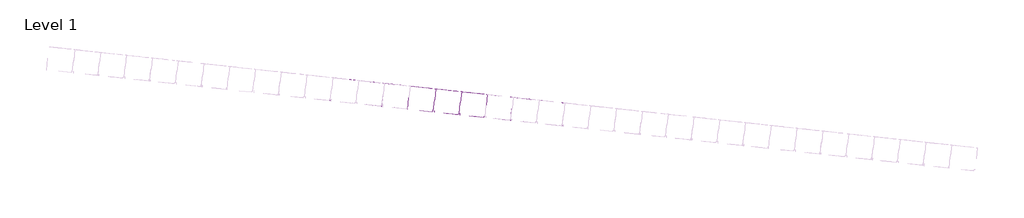
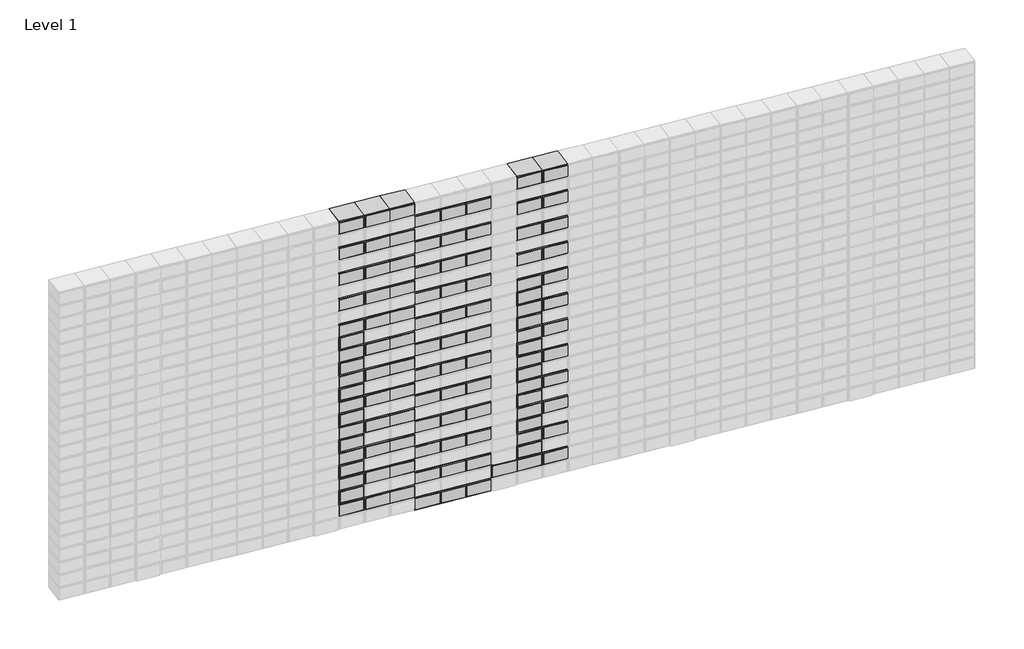
# One storey, part 14 of 18: 111 proxies.
"""IFC4 building model written with IfcOpenShell, lengths in millimetres."""

import ifcopenshell
import ifcopenshell.guid

model = None  # the IFC model being written
_history = None  # IfcOwnerHistory: only IFC2X3 demands one
_inside = {}  # id of a spatial element -> (the spatial element, [elements in it])
_under = {}  # id of a project, library or spatial element -> (it, [spatial elements below it])
_declared = {}  # id of a project -> (the project, [libraries it declares])
_typed = {}  # id of a type object -> (the type object, [elements of that type])
_made_of = {}  # id of a material, layer set ... -> (it, [elements and type objects made of it])


def new_model(schema):
    """Start an empty IFC model of exactly this schema.

    Asked for "IFC4X3", IfcOpenShell would pick the latest addendum, in which some entities
    have other attributes; the version numbers below select the first issue.
    IFC2X3 requires an IfcOwnerHistory on every rooted entity: one is made here for all.
    """
    global model, _history
    if schema == "IFC4X3":
        model = ifcopenshell.file(schema_version=(4, 3, 0, 0))
    else:
        model = ifcopenshell.file(schema=schema)
    _inside.clear()
    _under.clear()
    _declared.clear()
    _typed.clear()
    _made_of.clear()
    _history = None
    if model.schema == "IFC2X3":
        org = make("IfcOrganization", Name="unknown")
        user = make(
            "IfcPersonAndOrganization",
            ThePerson=make("IfcPerson", FamilyName="unknown"),
            TheOrganization=org,
        )
        app = make(
            "IfcApplication",
            ApplicationDeveloper=org,
            Version="unknown",
            ApplicationFullName="unknown",
            ApplicationIdentifier="unknown",
        )
        _history = make(
            "IfcOwnerHistory",
            OwningUser=user,
            OwningApplication=app,
            ChangeAction="ADDED",
            CreationDate=0,
        )
    return model


def make(cls, **values):
    """One entity of the class cls with the attributes given. An attribute that is None is left unset."""
    return model.create_entity(
        cls, **{name: value for name, value in values.items() if value is not None}
    )


def rooted(cls, **values):
    """An entity with a GlobalId (a new one), such as an element, a storey or a relation."""
    return make(cls, GlobalId=ifcopenshell.guid.new(), OwnerHistory=_history, **values)


def si_unit(unit_type, name, prefix=None):
    """IfcSIUnit, for example si_unit("LENGTHUNIT", "METRE", prefix="MILLI")."""
    return make("IfcSIUnit", UnitType=unit_type, Prefix=prefix, Name=name)


def assignment(units):
    """IfcUnitAssignment: the units of a project."""
    return None if units is None else make("IfcUnitAssignment", Units=units)


def point(xyz):
    """IfcCartesianPoint."""
    return None if xyz is None else make("IfcCartesianPoint", Coordinates=xyz)


def direction(xyz):
    """IfcDirection."""
    return None if xyz is None else make("IfcDirection", DirectionRatios=xyz)


def frame(location, z_axis=None, x_axis=None):
    """IfcAxis2Placement3D, a coordinate frame: its origin and axes. An axis left out is left unset."""
    return make(
        "IfcAxis2Placement3D",
        Location=point(location),
        Axis=direction(z_axis),
        RefDirection=direction(x_axis),
    )


def origin():
    """The frame at (0, 0, 0) with its axes left unset."""
    return frame((0.0, 0.0, 0.0))


def origin_with_axes():
    """The frame at (0, 0, 0) with the z axis (0, 0, 1) and the x axis (1, 0, 0) written out."""
    return frame((0.0, 0.0, 0.0), z_axis=(0.0, 0.0, 1.0), x_axis=(1.0, 0.0, 0.0))


def place(relative_to, where):
    """IfcLocalPlacement: puts the frame where relative to a parent placement (None: the world)."""
    return make(
        "IfcLocalPlacement", PlacementRelTo=relative_to, RelativePlacement=where
    )


def context(
    kind, dimensions, precision=None, world=None, true_north=None, identifier=None
):
    """IfcGeometricRepresentationContext, for example the 3D "Model" context."""
    return make(
        "IfcGeometricRepresentationContext",
        ContextIdentifier=identifier,
        ContextType=kind,
        CoordinateSpaceDimension=dimensions,
        Precision=precision,
        WorldCoordinateSystem=world,
        TrueNorth=true_north,
    )


def project(units=None, contexts=None):
    """IfcProject with its units and contexts."""
    return rooted(
        "IfcProject",
        Name="project",
        RepresentationContexts=contexts,
        UnitsInContext=assignment(units),
    )


def spatial(cls, under=None, at=None, **own):
    """A site, building, storey or space (cls), placed at a placement, below another one or the project."""
    s = rooted(cls, ObjectPlacement=at, **own)
    if under is not None:
        _under.setdefault(under.id(), (under, []))[1].append(s)
    return s


def polyline(points):
    """IfcPolyline through the points."""
    return make("IfcPolyline", Points=[point(p) for p in points])


def outline(outer, holes=None, kind="AREA"):
    """IfcArbitraryClosedProfileDef: a profile drawn as a closed curve; with holes, ...WithVoids."""
    if holes is None:
        return make("IfcArbitraryClosedProfileDef", ProfileType=kind, OuterCurve=outer)
    return make(
        "IfcArbitraryProfileDefWithVoids",
        ProfileType=kind,
        OuterCurve=outer,
        InnerCurves=holes,
    )


def extrude(swept, where, along, depth):
    """IfcExtrudedAreaSolid: the profile swept, set in the frame where, extruded along a direction by depth."""
    return make(
        "IfcExtrudedAreaSolid",
        SweptArea=swept,
        Position=where,
        ExtrudedDirection=direction(along),
        Depth=depth,
    )


def shape(context_of_items, identifier, shape_type, items):
    """IfcShapeRepresentation: the items that make up one representation, for example the "Body"."""
    return make(
        "IfcShapeRepresentation",
        ContextOfItems=context_of_items,
        RepresentationIdentifier=identifier,
        RepresentationType=shape_type,
        Items=items,
    )


def source(mapping_origin, context_of_items, identifier, shape_type, items):
    """IfcRepresentationMap: a shape defined once, which mapped items show again and again."""
    return make(
        "IfcRepresentationMap",
        MappingOrigin=mapping_origin,
        MappedRepresentation=shape(context_of_items, identifier, shape_type, items),
    )


def transform(
    local_origin,
    x_axis=None,
    y_axis=None,
    z_axis=None,
    scale=None,
    scale2=None,
    scale3=None,
    uniform=True,
):
    """IfcCartesianTransformationOperator3D, or its non-uniform kind. x_axis, y_axis, z_axis: its Axis1, 2, 3."""
    if uniform:
        return make(
            "IfcCartesianTransformationOperator3D",
            Axis1=direction(x_axis),
            Axis2=direction(y_axis),
            LocalOrigin=point(local_origin),
            Scale=scale,
            Axis3=direction(z_axis),
        )
    return make(
        "IfcCartesianTransformationOperator3DnonUniform",
        Axis1=direction(x_axis),
        Axis2=direction(y_axis),
        LocalOrigin=point(local_origin),
        Scale=scale,
        Axis3=direction(z_axis),
        Scale2=scale2,
        Scale3=scale3,
    )


def mapped(mapping_source, mapping_target):
    """IfcMappedItem: shows the shape of a source again, moved by a transform."""
    return make(
        "IfcMappedItem", MappingSource=mapping_source, MappingTarget=mapping_target
    )


def made_of(thing, what):
    """Note that an element or type object is made of a material, layer set ...; save() writes the relation."""
    if what is not None:
        _made_of.setdefault(what.id(), (what, []))[1].append(thing)
    return thing


def element(
    cls,
    number,
    at=None,
    inside=None,
    cuts=None,
    type_object=None,
    material=None,
    context=None,
    identifier="Body",
    shape_type=None,
    held_by="IfcProductDefinitionShape",
    body=None,
    shapes=None,
    **own,
):
    """One element of the class cls, such as IfcWall. Its Tag is "e" and its number.

    at: its placement. inside: the storey or other place that contains it. cuts: it is an
    opening in that element (IfcRelVoidsElement). A single representation is given by context,
    identifier, shape_type and body (its items); several are given by shapes. held_by: the class
    of the entity that holds the representations. save() writes the other relations.
    """
    e = rooted(cls, Tag="e%d" % number, ObjectPlacement=at, **own)
    if body is not None:
        shapes = [shape(context, identifier, shape_type, body)]
    if shapes is not None:
        e.Representation = make(held_by, Representations=shapes)
    if inside is not None:
        _inside.setdefault(inside.id(), (inside, []))[1].append(e)
    if cuts is not None:
        rooted(
            "IfcRelVoidsElement", RelatingBuildingElement=cuts, RelatedOpeningElement=e
        )
    if type_object is not None:
        _typed.setdefault(type_object.id(), (type_object, []))[1].append(e)
    return made_of(e, material)


def aggregate(whole, parts):
    """IfcRelAggregates: a whole, such as a stair, and the parts it consists of."""
    return rooted("IfcRelAggregates", RelatingObject=whole, RelatedObjects=parts)


def save(model, path):
    """Write the relations noted so far, then the file.

    IfcRelAggregates (storeys below a building ...), IfcRelContainedInSpatialStructure (elements
    in a storey), IfcRelDefinesByType, IfcRelAssociatesMaterial and IfcRelDeclares: one each for
    every whole, place, type object, material and project.
    """
    for whole, parts in _under.values():
        aggregate(whole, parts)
    for where, things in _inside.values():
        rooted(
            "IfcRelContainedInSpatialStructure",
            RelatedElements=things,
            RelatingStructure=where,
        )
    for kind, things in _typed.values():
        rooted("IfcRelDefinesByType", RelatedObjects=things, RelatingType=kind)
    for what, things in _made_of.values():
        rooted("IfcRelAssociatesMaterial", RelatedObjects=things, RelatingMaterial=what)
    for by, libraries in _declared.values():
        rooted("IfcRelDeclares", RelatingContext=by, RelatedDefinitions=libraries)
    model.write(path)


def geel_a5fc7152(model_context):
    return source(origin(), model_context, "Body", "SweptSolid", [
        extrude(outline(polyline([(131.1871262, 51.8695461), (24.8461542, 24.0369432), (23.5801491, 28.8740117), (125.0840527, 55.4406095), (111.9430518, 105.6488784), (10.4391482, 79.0822806), (9.1731432, 83.919349), (115.5141152, 111.7519519), (131.1871262, 51.8695461)])), origin_with_axes(), (0.0, 0.0, 1.0), 95.0),
        extrude(outline(polyline([(111.9430518, 105.6488784), (125.0840527, 55.4406095), (23.5801491, 28.8740117), (10.4391482, 79.0822806), (111.9430518, 105.6488784)])), origin_with_axes(), (0.0, 0.0, 1.0), 100.0),
    ])


def geel_ff5a4212(model_context):
    return source(origin(), model_context, "Body", "SweptSolid", [
        extrude(outline(polyline([(24.8461542, 24.0369432), (9.1731432, 83.919349), (115.5141152, 111.7519519), (116.7801202, 106.9148835), (15.2762167, 80.3482856), (28.4172176, 30.1400167), (129.9211211, 56.7066146), (131.1871262, 51.8695461), (24.8461542, 24.0369432)])), origin_with_axes(), (0.0, 0.0, 1.0), 95.0),
        extrude(outline(polyline([(116.7801202, 106.9148835), (129.9211211, 56.7066146), (28.4172176, 30.1400167), (15.2762167, 80.3482856), (116.7801202, 106.9148835)])), origin_with_axes(), (0.0, 0.0, 1.0), 100.0),
    ])


def rood_14a66368(model_context):
    return source(origin(), model_context, "Body", "SweptSolid", [
        extrude(outline(polyline([(24.8461542, 24.0369432), (9.1731432, 83.919349), (115.5141152, 111.7519519), (131.1871262, 51.8695461), (24.8461542, 24.0369432)]), holes=[polyline([(125.0840527, 55.4406095), (111.9430518, 105.6488784), (15.2762167, 80.3482856), (28.4172176, 30.1400167), (125.0840527, 55.4406095)])]), origin_with_axes(), (0.0, 0.0, 1.0), 95.0),
        extrude(outline(polyline([(111.9430518, 105.6488784), (125.0840527, 55.4406095), (28.4172176, 30.1400167), (15.2762167, 80.3482856), (111.9430518, 105.6488784)])), origin_with_axes(), (0.0, 0.0, 1.0), 100.0),
    ])


model = new_model("IFC4")

# Units and contexts
model_context = context("Model", 3, world=origin())
ifc_project = project(units=[si_unit("LENGTHUNIT", "METRE", prefix="MILLI")], contexts=[model_context])

# Site, building, storey
site = spatial("IfcSite", under=ifc_project)
building = spatial("IfcBuilding", under=site)
storey = spatial("IfcBuildingStorey", under=building, Name="Level 1", Elevation=0.0)

# Proxies
placement = place(None, origin())
geel_shape = geel_a5fc7152(model_context)
element("IfcBuildingElementProxy", 1, Name="Geel", ObjectType="Geel", at=placement, inside=storey, context=model_context, shape_type="MappedRepresentation", body=[
    mapped(geel_shape, transform((10079.135101, -4407.170809, 2168.7358475), x_axis=(0.9617275503729381, -0.10473475661476775, -0.25320100633787634), y_axis=(0.2517127736886919, -0.02741220845642843, 0.9674136914420257), z_axis=(-0.1082626362860859, -0.9941223272738555, 0.0))),
])
element("IfcBuildingElementProxy", 2, Name="Geel", ObjectType="Geel", at=placement, inside=storey, context=model_context, shape_type="MappedRepresentation", body=[
    mapped(geel_shape, transform((10844.0731503, -4490.4746516, 2168.7358475), x_axis=(0.9617275503729374, -0.1047347566147725, -0.25320100633787673), y_axis=(0.25171277368869216, -0.02741220845642974, 0.9674136914420255), z_axis=(-0.10826263628609081, -0.9941223272738551, 0.0))),
])
element("IfcBuildingElementProxy", 3, Name="Geel", ObjectType="Geel", at=placement, inside=storey, context=model_context, shape_type="MappedRepresentation", body=[
    mapped(geel_shape, transform((10079.135101, -4407.170809, 2292.5348104), x_axis=(0.9617275503729381, -0.10473475661476775, -0.25320100633787634), y_axis=(0.2517127736886919, -0.02741220845642843, 0.9674136914420257), z_axis=(-0.1082626362860859, -0.9941223272738555, 0.0))),
])
element("IfcBuildingElementProxy", 4, Name="Geel", ObjectType="Geel", at=placement, inside=storey, context=model_context, shape_type="MappedRepresentation", body=[
    mapped(geel_shape, transform((10844.0731503, -4490.4746516, 2292.5348104), x_axis=(0.9617275503729374, -0.1047347566147725, -0.25320100633787673), y_axis=(0.25171277368869216, -0.02741220845642974, 0.9674136914420255), z_axis=(-0.10826263628609081, -0.9941223272738551, 0.0))),
])
element("IfcBuildingElementProxy", 5, Name="Geel", ObjectType="Geel", at=placement, inside=storey, context=model_context, shape_type="MappedRepresentation", body=[
    mapped(geel_shape, transform((10079.135101, -4407.170809, 2416.3337732), x_axis=(0.961727550372939, -0.10473475661476785, -0.2532010063378727), y_axis=(0.2517127736886882, -0.02741220845642804, 0.9674136914420266), z_axis=(-0.1082626362860859, -0.9941223272738555, 0.0))),
])
element("IfcBuildingElementProxy", 6, Name="Geel", ObjectType="Geel", at=placement, inside=storey, context=model_context, shape_type="MappedRepresentation", body=[
    mapped(geel_shape, transform((10844.0731503, -4490.4746516, 2416.3337732), x_axis=(0.9617275503729384, -0.1047347566147726, -0.25320100633787307), y_axis=(0.25171277368868855, -0.02741220845642934, 0.9674136914420265), z_axis=(-0.10826263628609081, -0.994122327273855, 0.0))),
])
element("IfcBuildingElementProxy", 7, Name="Geel", ObjectType="Geel", at=placement, inside=storey, context=model_context, shape_type="MappedRepresentation", body=[
    mapped(geel_shape, transform((10079.135101, -4407.170809, 2540.132736), x_axis=(0.9617275503729381, -0.10473475661476775, -0.25320100633787634), y_axis=(0.2517127736886919, -0.02741220845642843, 0.9674136914420257), z_axis=(-0.1082626362860859, -0.9941223272738555, 0.0))),
])
element("IfcBuildingElementProxy", 8, Name="Geel", ObjectType="Geel", at=placement, inside=storey, context=model_context, shape_type="MappedRepresentation", body=[
    mapped(geel_shape, transform((10844.0731503, -4490.4746516, 2540.132736), x_axis=(0.9617275503729374, -0.1047347566147725, -0.25320100633787673), y_axis=(0.25171277368869216, -0.02741220845642974, 0.9674136914420255), z_axis=(-0.10826263628609081, -0.9941223272738551, 0.0))),
])
element("IfcBuildingElementProxy", 9, Name="Geel", ObjectType="Geel", at=placement, inside=storey, context=model_context, shape_type="MappedRepresentation", body=[
    mapped(geel_shape, transform((10079.135101, -4407.170809, 2663.9316989), x_axis=(0.9617275503729381, -0.10473475661476775, -0.25320100633787634), y_axis=(0.2517127736886919, -0.02741220845642843, 0.9674136914420257), z_axis=(-0.1082626362860859, -0.9941223272738555, 0.0))),
])
element("IfcBuildingElementProxy", 10, Name="Geel", ObjectType="Geel", at=placement, inside=storey, context=model_context, shape_type="MappedRepresentation", body=[
    mapped(geel_shape, transform((10844.0731503, -4490.4746516, 2663.9316989), x_axis=(0.9617275503729374, -0.1047347566147725, -0.25320100633787673), y_axis=(0.25171277368869216, -0.02741220845642974, 0.9674136914420255), z_axis=(-0.10826263628609081, -0.9941223272738551, 0.0))),
])
element("IfcBuildingElementProxy", 11, Name="Geel", ObjectType="Geel", at=placement, inside=storey, context=model_context, shape_type="MappedRepresentation", body=[
    mapped(geel_shape, transform((10079.135101, -4407.170809, 2787.7306617), x_axis=(0.9617275503729381, -0.10473475661476775, -0.25320100633787634), y_axis=(0.2517127736886919, -0.02741220845642843, 0.9674136914420257), z_axis=(-0.1082626362860859, -0.9941223272738555, 0.0))),
])
element("IfcBuildingElementProxy", 12, Name="Geel", ObjectType="Geel", at=placement, inside=storey, context=model_context, shape_type="MappedRepresentation", body=[
    mapped(geel_shape, transform((10844.0731503, -4490.4746516, 2787.7306617), x_axis=(0.9617275503729374, -0.1047347566147725, -0.25320100633787673), y_axis=(0.25171277368869216, -0.02741220845642974, 0.9674136914420255), z_axis=(-0.10826263628609081, -0.9941223272738551, 0.0))),
])
element("IfcBuildingElementProxy", 13, Name="Geel", ObjectType="Geel", at=placement, inside=storey, context=model_context, shape_type="MappedRepresentation", body=[
    mapped(geel_shape, transform((10079.135101, -4407.170809, 2911.5296245), x_axis=(0.9617275503729381, -0.10473475661476775, -0.25320100633787634), y_axis=(0.2517127736886919, -0.02741220845642843, 0.9674136914420257), z_axis=(-0.1082626362860859, -0.9941223272738555, 0.0))),
])
element("IfcBuildingElementProxy", 14, Name="Geel", ObjectType="Geel", at=placement, inside=storey, context=model_context, shape_type="MappedRepresentation", body=[
    mapped(geel_shape, transform((10844.0731503, -4490.4746516, 2911.5296245), x_axis=(0.9617275503729374, -0.1047347566147725, -0.25320100633787673), y_axis=(0.25171277368869216, -0.02741220845642974, 0.9674136914420255), z_axis=(-0.10826263628609081, -0.9941223272738551, 0.0))),
])
element("IfcBuildingElementProxy", 15, Name="Geel", ObjectType="Geel", at=placement, inside=storey, context=model_context, shape_type="MappedRepresentation", body=[
    mapped(geel_shape, transform((10079.135101, -4407.170809, 3035.3285874), x_axis=(0.9617275503729381, -0.10473475661476775, -0.25320100633787634), y_axis=(0.2517127736886919, -0.02741220845642843, 0.9674136914420257), z_axis=(-0.1082626362860859, -0.9941223272738555, 0.0))),
])
element("IfcBuildingElementProxy", 16, Name="Geel", ObjectType="Geel", at=placement, inside=storey, context=model_context, shape_type="MappedRepresentation", body=[
    mapped(geel_shape, transform((10844.0731503, -4490.4746516, 3035.3285874), x_axis=(0.9617275503729374, -0.1047347566147725, -0.25320100633787673), y_axis=(0.25171277368869216, -0.02741220845642974, 0.9674136914420255), z_axis=(-0.10826263628609081, -0.9941223272738551, 0.0))),
])
element("IfcBuildingElementProxy", 17, Name="Geel", ObjectType="Geel", at=placement, inside=storey, context=model_context, shape_type="MappedRepresentation", body=[
    mapped(geel_shape, transform((10079.135101, -4407.170809, 3159.1275502), x_axis=(0.9617275503729381, -0.10473475661476775, -0.25320100633787634), y_axis=(0.2517127736886919, -0.02741220845642843, 0.9674136914420257), z_axis=(-0.1082626362860859, -0.9941223272738555, 0.0))),
])
element("IfcBuildingElementProxy", 18, Name="Geel", ObjectType="Geel", at=placement, inside=storey, context=model_context, shape_type="MappedRepresentation", body=[
    mapped(geel_shape, transform((10844.0731503, -4490.4746516, 3159.1275502), x_axis=(0.9617275503729374, -0.1047347566147725, -0.25320100633787673), y_axis=(0.25171277368869216, -0.02741220845642974, 0.9674136914420255), z_axis=(-0.10826263628609081, -0.9941223272738551, 0.0))),
])
element("IfcBuildingElementProxy", 19, Name="Geel", ObjectType="Geel", at=placement, inside=storey, context=model_context, shape_type="MappedRepresentation", body=[
    mapped(geel_shape, transform((10079.135101, -4407.170809, 3282.926513), x_axis=(0.9617275503729381, -0.10473475661476775, -0.25320100633787634), y_axis=(0.2517127736886919, -0.02741220845642843, 0.9674136914420257), z_axis=(-0.1082626362860859, -0.9941223272738555, 0.0))),
])
element("IfcBuildingElementProxy", 20, Name="Geel", ObjectType="Geel", at=placement, inside=storey, context=model_context, shape_type="MappedRepresentation", body=[
    mapped(geel_shape, transform((10844.0731503, -4490.4746516, 3282.926513), x_axis=(0.9617275503729374, -0.1047347566147725, -0.25320100633787673), y_axis=(0.25171277368869216, -0.02741220845642974, 0.9674136914420255), z_axis=(-0.10826263628609081, -0.9941223272738551, 0.0))),
])
element("IfcBuildingElementProxy", 21, Name="Geel", ObjectType="Geel", at=placement, inside=storey, context=model_context, shape_type="MappedRepresentation", body=[
    mapped(geel_shape, transform((10079.135101, -4407.170809, 3406.7254759), x_axis=(0.9617275503729381, -0.10473475661476775, -0.25320100633787634), y_axis=(0.2517127736886919, -0.02741220845642843, 0.9674136914420257), z_axis=(-0.1082626362860859, -0.9941223272738555, 0.0))),
])
element("IfcBuildingElementProxy", 22, Name="Geel", ObjectType="Geel", at=placement, inside=storey, context=model_context, shape_type="MappedRepresentation", body=[
    mapped(geel_shape, transform((10844.0731503, -4490.4746516, 3406.7254759), x_axis=(0.9617275503729374, -0.1047347566147725, -0.25320100633787673), y_axis=(0.25171277368869216, -0.02741220845642974, 0.9674136914420255), z_axis=(-0.10826263628609081, -0.9941223272738551, 0.0))),
])
element("IfcBuildingElementProxy", 23, Name="Geel", ObjectType="Geel", at=placement, inside=storey, context=model_context, shape_type="MappedRepresentation", body=[
    mapped(geel_shape, transform((10079.135101, -4407.170809, 2044.9368847), x_axis=(0.961727550372939, -0.10473475661476785, -0.2532010063378727), y_axis=(0.2517127736886882, -0.02741220845642804, 0.9674136914420266), z_axis=(-0.1082626362860859, -0.9941223272738555, 0.0))),
])
element("IfcBuildingElementProxy", 24, Name="Geel", ObjectType="Geel", at=placement, inside=storey, context=model_context, shape_type="MappedRepresentation", body=[
    mapped(geel_shape, transform((10844.0731503, -4490.4746516, 2044.9368847), x_axis=(0.9617275503729384, -0.1047347566147726, -0.25320100633787307), y_axis=(0.25171277368868855, -0.02741220845642934, 0.9674136914420265), z_axis=(-0.10826263628609081, -0.994122327273855, 0.0))),
])
element("IfcBuildingElementProxy", 25, Name="Geel", ObjectType="Geel", at=placement, inside=storey, context=model_context, shape_type="MappedRepresentation", body=[
    mapped(geel_shape, transform((10297.6888294, -4430.9719069, 2168.7358475), x_axis=(0.9617275503729374, -0.1047347566147725, -0.25320100633787673), y_axis=(0.25171277368869216, -0.02741220845642974, 0.9674136914420255), z_axis=(-0.10826263628609081, -0.9941223272738551, 0.0))),
])
element("IfcBuildingElementProxy", 26, Name="Geel", ObjectType="Geel", at=placement, inside=storey, context=model_context, shape_type="MappedRepresentation", body=[
    mapped(geel_shape, transform((10297.6888294, -4430.9719069, 2292.5348104), x_axis=(0.9617275503729374, -0.1047347566147725, -0.25320100633787673), y_axis=(0.25171277368869216, -0.02741220845642974, 0.9674136914420255), z_axis=(-0.10826263628609081, -0.9941223272738551, 0.0))),
])
element("IfcBuildingElementProxy", 27, Name="Geel", ObjectType="Geel", at=placement, inside=storey, context=model_context, shape_type="MappedRepresentation", body=[
    mapped(geel_shape, transform((10297.6888294, -4430.9719069, 2416.3337732), x_axis=(0.9617275503729384, -0.1047347566147726, -0.25320100633787307), y_axis=(0.25171277368868855, -0.02741220845642934, 0.9674136914420265), z_axis=(-0.10826263628609081, -0.994122327273855, 0.0))),
])
element("IfcBuildingElementProxy", 28, Name="Geel", ObjectType="Geel", at=placement, inside=storey, context=model_context, shape_type="MappedRepresentation", body=[
    mapped(geel_shape, transform((10297.6888294, -4430.9719069, 2540.132736), x_axis=(0.9617275503729374, -0.1047347566147725, -0.25320100633787673), y_axis=(0.25171277368869216, -0.02741220845642974, 0.9674136914420255), z_axis=(-0.10826263628609081, -0.9941223272738551, 0.0))),
])
element("IfcBuildingElementProxy", 29, Name="Geel", ObjectType="Geel", at=placement, inside=storey, context=model_context, shape_type="MappedRepresentation", body=[
    mapped(geel_shape, transform((10297.6888294, -4430.9719069, 2663.9316989), x_axis=(0.9617275503729374, -0.1047347566147725, -0.25320100633787673), y_axis=(0.25171277368869216, -0.02741220845642974, 0.9674136914420255), z_axis=(-0.10826263628609081, -0.9941223272738551, 0.0))),
])
element("IfcBuildingElementProxy", 30, Name="Geel", ObjectType="Geel", at=placement, inside=storey, context=model_context, shape_type="MappedRepresentation", body=[
    mapped(geel_shape, transform((10297.6888294, -4430.9719069, 2787.7306617), x_axis=(0.9617275503729374, -0.1047347566147725, -0.25320100633787673), y_axis=(0.25171277368869216, -0.02741220845642974, 0.9674136914420255), z_axis=(-0.10826263628609081, -0.9941223272738551, 0.0))),
])
element("IfcBuildingElementProxy", 31, Name="Geel", ObjectType="Geel", at=placement, inside=storey, context=model_context, shape_type="MappedRepresentation", body=[
    mapped(geel_shape, transform((10297.6888294, -4430.9719069, 2911.5296245), x_axis=(0.9617275503729374, -0.1047347566147725, -0.25320100633787673), y_axis=(0.25171277368869216, -0.02741220845642974, 0.9674136914420255), z_axis=(-0.10826263628609081, -0.9941223272738551, 0.0))),
])
element("IfcBuildingElementProxy", 32, Name="Geel", ObjectType="Geel", at=placement, inside=storey, context=model_context, shape_type="MappedRepresentation", body=[
    mapped(geel_shape, transform((10297.6888294, -4430.9719069, 3035.3285874), x_axis=(0.9617275503729374, -0.1047347566147725, -0.25320100633787673), y_axis=(0.25171277368869216, -0.02741220845642974, 0.9674136914420255), z_axis=(-0.10826263628609081, -0.9941223272738551, 0.0))),
])
element("IfcBuildingElementProxy", 33, Name="Geel", ObjectType="Geel", at=placement, inside=storey, context=model_context, shape_type="MappedRepresentation", body=[
    mapped(geel_shape, transform((10297.6888294, -4430.9719069, 3159.1275502), x_axis=(0.9617275503729374, -0.1047347566147725, -0.25320100633787673), y_axis=(0.25171277368869216, -0.02741220845642974, 0.9674136914420255), z_axis=(-0.10826263628609081, -0.9941223272738551, 0.0))),
])
element("IfcBuildingElementProxy", 34, Name="Geel", ObjectType="Geel", at=placement, inside=storey, context=model_context, shape_type="MappedRepresentation", body=[
    mapped(geel_shape, transform((10297.6888294, -4430.9719069, 3282.926513), x_axis=(0.9617275503729374, -0.1047347566147725, -0.25320100633787673), y_axis=(0.25171277368869216, -0.02741220845642974, 0.9674136914420255), z_axis=(-0.10826263628609081, -0.9941223272738551, 0.0))),
])
element("IfcBuildingElementProxy", 35, Name="Geel", ObjectType="Geel", at=placement, inside=storey, context=model_context, shape_type="MappedRepresentation", body=[
    mapped(geel_shape, transform((10297.6888294, -4430.9719069, 3406.7254759), x_axis=(0.9617275503729374, -0.1047347566147725, -0.25320100633787673), y_axis=(0.25171277368869216, -0.02741220845642974, 0.9674136914420255), z_axis=(-0.10826263628609081, -0.9941223272738551, 0.0))),
])
element("IfcBuildingElementProxy", 36, Name="Geel", ObjectType="Geel", at=placement, inside=storey, context=model_context, shape_type="MappedRepresentation", body=[
    mapped(geel_shape, transform((10297.6888294, -4430.9719069, 2044.9368847), x_axis=(0.9617275503729384, -0.1047347566147726, -0.25320100633787307), y_axis=(0.25171277368868855, -0.02741220845642934, 0.9674136914420265), z_axis=(-0.10826263628609081, -0.994122327273855, 0.0))),
])
geel_2_shape = geel_ff5a4212(model_context)
element("IfcBuildingElementProxy", 37, Name="Geel", ObjectType="Geel", at=placement, inside=storey, context=model_context, shape_type="MappedRepresentation", body=[
    mapped(geel_2_shape, transform((10734.7962861, -4478.5741026, 2044.9368847), x_axis=(0.961727550372943, -0.10473475661477039, -0.25320100633785686), y_axis=(0.25171277368867245, -0.02741220845642689, 0.9674136914420308), z_axis=(-0.10826263628608805, -0.9941223272738553, 0.0))),
])
element("IfcBuildingElementProxy", 38, Name="Geel", ObjectType="Geel", at=placement, inside=storey, context=model_context, shape_type="MappedRepresentation", body=[
    mapped(geel_2_shape, transform((10188.4119652, -4419.071358, 2168.7358475), x_axis=(0.9617275503729416, -0.10473475661477503, -0.2532010063378606), y_axis=(0.25171277368867595, -0.027412208456428513, 0.9674136914420297), z_axis=(-0.10826263628609296, -0.9941223272738547, 0.0))),
])
element("IfcBuildingElementProxy", 39, Name="Geel", ObjectType="Geel", at=placement, inside=storey, context=model_context, shape_type="MappedRepresentation", body=[
    mapped(geel_2_shape, transform((10953.3500145, -4502.3752005, 2168.7358475), x_axis=(0.961727550372942, -0.10473475661477023, -0.25320100633786047), y_axis=(0.2517127736886762, -0.02741220845642727, 0.9674136914420297), z_axis=(-0.10826263628608801, -0.9941223272738554, 0.0))),
])
element("IfcBuildingElementProxy", 40, Name="Geel", ObjectType="Geel", at=placement, inside=storey, context=model_context, shape_type="MappedRepresentation", body=[
    mapped(geel_2_shape, transform((10188.4119652, -4419.071358, 2292.5348104), x_axis=(0.9617275503729416, -0.10473475661477503, -0.2532010063378606), y_axis=(0.25171277368867595, -0.027412208456428513, 0.9674136914420297), z_axis=(-0.10826263628609296, -0.9941223272738547, 0.0))),
])
element("IfcBuildingElementProxy", 41, Name="Geel", ObjectType="Geel", at=placement, inside=storey, context=model_context, shape_type="MappedRepresentation", body=[
    mapped(geel_2_shape, transform((10953.3500145, -4502.3752005, 2292.5348104), x_axis=(0.961727550372942, -0.10473475661477023, -0.25320100633786047), y_axis=(0.2517127736886762, -0.02741220845642727, 0.9674136914420297), z_axis=(-0.10826263628608801, -0.9941223272738554, 0.0))),
])
element("IfcBuildingElementProxy", 42, Name="Geel", ObjectType="Geel", at=placement, inside=storey, context=model_context, shape_type="MappedRepresentation", body=[
    mapped(geel_2_shape, transform((10188.4119652, -4419.071358, 2416.3337732), x_axis=(0.9617275503729426, -0.10473475661477512, -0.253201006337857), y_axis=(0.2517127736886723, -0.027412208456428104, 0.9674136914420308), z_axis=(-0.10826263628609295, -0.9941223272738549, 0.0))),
])
element("IfcBuildingElementProxy", 43, Name="Geel", ObjectType="Geel", at=placement, inside=storey, context=model_context, shape_type="MappedRepresentation", body=[
    mapped(geel_2_shape, transform((10953.3500145, -4502.3752005, 2416.3337732), x_axis=(0.961727550372943, -0.10473475661477034, -0.25320100633785686), y_axis=(0.25171277368867245, -0.027412208456426876, 0.9674136914420308), z_axis=(-0.10826263628608801, -0.9941223272738553, 0.0))),
])
element("IfcBuildingElementProxy", 44, Name="Geel", ObjectType="Geel", at=placement, inside=storey, context=model_context, shape_type="MappedRepresentation", body=[
    mapped(geel_2_shape, transform((10188.4119652, -4419.071358, 2540.132736), x_axis=(0.9617275503729416, -0.10473475661477503, -0.2532010063378606), y_axis=(0.25171277368867595, -0.027412208456428513, 0.9674136914420297), z_axis=(-0.10826263628609296, -0.9941223272738547, 0.0))),
])
element("IfcBuildingElementProxy", 45, Name="Geel", ObjectType="Geel", at=placement, inside=storey, context=model_context, shape_type="MappedRepresentation", body=[
    mapped(geel_2_shape, transform((10953.3500145, -4502.3752005, 2540.132736), x_axis=(0.961727550372942, -0.10473475661477023, -0.25320100633786047), y_axis=(0.2517127736886762, -0.02741220845642727, 0.9674136914420297), z_axis=(-0.10826263628608801, -0.9941223272738554, 0.0))),
])
element("IfcBuildingElementProxy", 46, Name="Geel", ObjectType="Geel", at=placement, inside=storey, context=model_context, shape_type="MappedRepresentation", body=[
    mapped(geel_2_shape, transform((10188.4119652, -4419.071358, 2663.9316989), x_axis=(0.9617275503729416, -0.10473475661477503, -0.2532010063378606), y_axis=(0.25171277368867595, -0.027412208456428513, 0.9674136914420297), z_axis=(-0.10826263628609296, -0.9941223272738547, 0.0))),
])
element("IfcBuildingElementProxy", 47, Name="Geel", ObjectType="Geel", at=placement, inside=storey, context=model_context, shape_type="MappedRepresentation", body=[
    mapped(geel_2_shape, transform((10953.3500145, -4502.3752005, 2663.9316989), x_axis=(0.961727550372942, -0.10473475661477023, -0.25320100633786047), y_axis=(0.2517127736886762, -0.02741220845642727, 0.9674136914420297), z_axis=(-0.10826263628608801, -0.9941223272738554, 0.0))),
])
element("IfcBuildingElementProxy", 48, Name="Geel", ObjectType="Geel", at=placement, inside=storey, context=model_context, shape_type="MappedRepresentation", body=[
    mapped(geel_2_shape, transform((10188.4119652, -4419.071358, 2787.7306617), x_axis=(0.9617275503729416, -0.10473475661477503, -0.2532010063378606), y_axis=(0.25171277368867595, -0.027412208456428513, 0.9674136914420297), z_axis=(-0.10826263628609296, -0.9941223272738547, 0.0))),
])
element("IfcBuildingElementProxy", 49, Name="Geel", ObjectType="Geel", at=placement, inside=storey, context=model_context, shape_type="MappedRepresentation", body=[
    mapped(geel_2_shape, transform((10953.3500145, -4502.3752005, 2787.7306617), x_axis=(0.961727550372942, -0.10473475661477023, -0.25320100633786047), y_axis=(0.2517127736886762, -0.02741220845642727, 0.9674136914420297), z_axis=(-0.10826263628608801, -0.9941223272738554, 0.0))),
])
element("IfcBuildingElementProxy", 50, Name="Geel", ObjectType="Geel", at=placement, inside=storey, context=model_context, shape_type="MappedRepresentation", body=[
    mapped(geel_2_shape, transform((10188.4119652, -4419.071358, 2911.5296245), x_axis=(0.9617275503729416, -0.10473475661477503, -0.2532010063378606), y_axis=(0.25171277368867595, -0.027412208456428513, 0.9674136914420297), z_axis=(-0.10826263628609296, -0.9941223272738547, 0.0))),
])
element("IfcBuildingElementProxy", 51, Name="Geel", ObjectType="Geel", at=placement, inside=storey, context=model_context, shape_type="MappedRepresentation", body=[
    mapped(geel_2_shape, transform((10953.3500145, -4502.3752005, 2911.5296245), x_axis=(0.961727550372942, -0.10473475661477023, -0.25320100633786047), y_axis=(0.2517127736886762, -0.02741220845642727, 0.9674136914420297), z_axis=(-0.10826263628608801, -0.9941223272738554, 0.0))),
])
element("IfcBuildingElementProxy", 52, Name="Geel", ObjectType="Geel", at=placement, inside=storey, context=model_context, shape_type="MappedRepresentation", body=[
    mapped(geel_2_shape, transform((10188.4119652, -4419.071358, 3035.3285874), x_axis=(0.9617275503729416, -0.10473475661477503, -0.2532010063378606), y_axis=(0.25171277368867595, -0.027412208456428513, 0.9674136914420297), z_axis=(-0.10826263628609296, -0.9941223272738547, 0.0))),
])
element("IfcBuildingElementProxy", 53, Name="Geel", ObjectType="Geel", at=placement, inside=storey, context=model_context, shape_type="MappedRepresentation", body=[
    mapped(geel_2_shape, transform((10953.3500145, -4502.3752005, 3035.3285874), x_axis=(0.961727550372942, -0.10473475661477023, -0.25320100633786047), y_axis=(0.2517127736886762, -0.02741220845642727, 0.9674136914420297), z_axis=(-0.10826263628608801, -0.9941223272738554, 0.0))),
])
element("IfcBuildingElementProxy", 54, Name="Geel", ObjectType="Geel", at=placement, inside=storey, context=model_context, shape_type="MappedRepresentation", body=[
    mapped(geel_2_shape, transform((10188.4119652, -4419.071358, 3159.1275502), x_axis=(0.9617275503729416, -0.10473475661477503, -0.2532010063378606), y_axis=(0.25171277368867595, -0.027412208456428513, 0.9674136914420297), z_axis=(-0.10826263628609296, -0.9941223272738547, 0.0))),
])
element("IfcBuildingElementProxy", 55, Name="Geel", ObjectType="Geel", at=placement, inside=storey, context=model_context, shape_type="MappedRepresentation", body=[
    mapped(geel_2_shape, transform((10953.3500145, -4502.3752005, 3159.1275502), x_axis=(0.961727550372942, -0.10473475661477023, -0.25320100633786047), y_axis=(0.2517127736886762, -0.02741220845642727, 0.9674136914420297), z_axis=(-0.10826263628608801, -0.9941223272738554, 0.0))),
])
element("IfcBuildingElementProxy", 56, Name="Geel", ObjectType="Geel", at=placement, inside=storey, context=model_context, shape_type="MappedRepresentation", body=[
    mapped(geel_2_shape, transform((10188.4119652, -4419.071358, 3282.926513), x_axis=(0.9617275503729416, -0.10473475661477503, -0.2532010063378606), y_axis=(0.25171277368867595, -0.027412208456428513, 0.9674136914420297), z_axis=(-0.10826263628609296, -0.9941223272738547, 0.0))),
])
element("IfcBuildingElementProxy", 57, Name="Geel", ObjectType="Geel", at=placement, inside=storey, context=model_context, shape_type="MappedRepresentation", body=[
    mapped(geel_2_shape, transform((10953.3500145, -4502.3752005, 3282.926513), x_axis=(0.961727550372942, -0.10473475661477023, -0.25320100633786047), y_axis=(0.2517127736886762, -0.02741220845642727, 0.9674136914420297), z_axis=(-0.10826263628608801, -0.9941223272738554, 0.0))),
])
element("IfcBuildingElementProxy", 58, Name="Geel", ObjectType="Geel", at=placement, inside=storey, context=model_context, shape_type="MappedRepresentation", body=[
    mapped(geel_2_shape, transform((10188.4119652, -4419.071358, 3406.7254759), x_axis=(0.9617275503729416, -0.10473475661477503, -0.2532010063378606), y_axis=(0.25171277368867595, -0.027412208456428513, 0.9674136914420297), z_axis=(-0.10826263628609296, -0.9941223272738547, 0.0))),
])
element("IfcBuildingElementProxy", 59, Name="Geel", ObjectType="Geel", at=placement, inside=storey, context=model_context, shape_type="MappedRepresentation", body=[
    mapped(geel_2_shape, transform((10953.3500145, -4502.3752005, 3406.7254759), x_axis=(0.961727550372942, -0.10473475661477023, -0.25320100633786047), y_axis=(0.2517127736886762, -0.02741220845642727, 0.9674136914420297), z_axis=(-0.10826263628608801, -0.9941223272738554, 0.0))),
])
element("IfcBuildingElementProxy", 60, Name="Geel", ObjectType="Geel", at=placement, inside=storey, context=model_context, shape_type="MappedRepresentation", body=[
    mapped(geel_2_shape, transform((10188.4119652, -4419.071358, 2044.9368847), x_axis=(0.9617275503729426, -0.10473475661477512, -0.253201006337857), y_axis=(0.2517127736886723, -0.027412208456428104, 0.9674136914420308), z_axis=(-0.10826263628609295, -0.9941223272738549, 0.0))),
])
element("IfcBuildingElementProxy", 61, Name="Geel", ObjectType="Geel", at=placement, inside=storey, context=model_context, shape_type="MappedRepresentation", body=[
    mapped(geel_2_shape, transform((10953.3500145, -4502.3752005, 2044.9368847), x_axis=(0.961727550372943, -0.10473475661477034, -0.25320100633785686), y_axis=(0.25171277368867245, -0.027412208456426876, 0.9674136914420308), z_axis=(-0.10826263628608801, -0.9941223272738553, 0.0))),
])
element("IfcBuildingElementProxy", 62, Name="Rood", ObjectType="Rood", at=placement, inside=storey, context=model_context, shape_type="MappedRepresentation", body=[
    mapped(geel_shape, transform((10406.9656935, -4442.8724558, 2106.8363661), x_axis=(0.9617275503729374, -0.1047347566147725, -0.25320100633787673), y_axis=(0.25171277368869216, -0.02741220845642974, 0.9674136914420255), z_axis=(-0.10826263628609081, -0.9941223272738551, 0.0))),
])
element("IfcBuildingElementProxy", 63, Name="Rood", ObjectType="Rood", at=placement, inside=storey, context=model_context, shape_type="MappedRepresentation", body=[
    mapped(geel_shape, transform((10406.9656935, -4442.8724558, 2230.6353289), x_axis=(0.9617275503729384, -0.1047347566147726, -0.25320100633787307), y_axis=(0.25171277368868855, -0.02741220845642934, 0.9674136914420265), z_axis=(-0.10826263628609081, -0.994122327273855, 0.0))),
])
element("IfcBuildingElementProxy", 64, Name="Rood", ObjectType="Rood", at=placement, inside=storey, context=model_context, shape_type="MappedRepresentation", body=[
    mapped(geel_shape, transform((10406.9656935, -4442.8724558, 2354.4342918), x_axis=(0.9617275503729374, -0.1047347566147725, -0.25320100633787673), y_axis=(0.25171277368869216, -0.02741220845642974, 0.9674136914420255), z_axis=(-0.10826263628609081, -0.9941223272738551, 0.0))),
])
element("IfcBuildingElementProxy", 65, Name="Rood", ObjectType="Rood", at=placement, inside=storey, context=model_context, shape_type="MappedRepresentation", body=[
    mapped(geel_shape, transform((10406.9656935, -4442.8724558, 2478.2332546), x_axis=(0.9617275503729374, -0.1047347566147725, -0.25320100633787673), y_axis=(0.25171277368869216, -0.02741220845642974, 0.9674136914420255), z_axis=(-0.10826263628609081, -0.9941223272738551, 0.0))),
])
element("IfcBuildingElementProxy", 66, Name="Rood", ObjectType="Rood", at=placement, inside=storey, context=model_context, shape_type="MappedRepresentation", body=[
    mapped(geel_shape, transform((10406.9656935, -4442.8724558, 2602.0322174), x_axis=(0.9617275503729394, -0.10473475661477268, -0.2532010063378695), y_axis=(0.2517127736886849, -0.027412208456428923, 0.9674136914420275), z_axis=(-0.1082626362860908, -0.9941223272738551, 0.0))),
])
element("IfcBuildingElementProxy", 67, Name="Rood", ObjectType="Rood", at=placement, inside=storey, context=model_context, shape_type="MappedRepresentation", body=[
    mapped(geel_shape, transform((10406.9656935, -4442.8724558, 2725.8311803), x_axis=(0.9617275503729374, -0.1047347566147725, -0.25320100633787673), y_axis=(0.25171277368869216, -0.02741220845642974, 0.9674136914420255), z_axis=(-0.10826263628609081, -0.9941223272738551, 0.0))),
])
element("IfcBuildingElementProxy", 68, Name="Rood", ObjectType="Rood", at=placement, inside=storey, context=model_context, shape_type="MappedRepresentation", body=[
    mapped(geel_shape, transform((10406.9656935, -4442.8724558, 2849.6301431), x_axis=(0.9617275503729374, -0.1047347566147725, -0.25320100633787673), y_axis=(0.25171277368869216, -0.02741220845642974, 0.9674136914420255), z_axis=(-0.10826263628609081, -0.9941223272738551, 0.0))),
])
element("IfcBuildingElementProxy", 69, Name="Rood", ObjectType="Rood", at=placement, inside=storey, context=model_context, shape_type="MappedRepresentation", body=[
    mapped(geel_shape, transform((10406.9656935, -4442.8724558, 2973.4291059), x_axis=(0.9617275503729374, -0.1047347566147725, -0.25320100633787673), y_axis=(0.25171277368869216, -0.02741220845642974, 0.9674136914420255), z_axis=(-0.10826263628609081, -0.9941223272738551, 0.0))),
])
element("IfcBuildingElementProxy", 70, Name="Rood", ObjectType="Rood", at=placement, inside=storey, context=model_context, shape_type="MappedRepresentation", body=[
    mapped(geel_shape, transform((10406.9656935, -4442.8724558, 3097.2280688), x_axis=(0.9617275503729394, -0.10473475661477268, -0.2532010063378695), y_axis=(0.2517127736886849, -0.027412208456428923, 0.9674136914420275), z_axis=(-0.1082626362860908, -0.9941223272738551, 0.0))),
])
element("IfcBuildingElementProxy", 71, Name="Rood", ObjectType="Rood", at=placement, inside=storey, context=model_context, shape_type="MappedRepresentation", body=[
    mapped(geel_shape, transform((10406.9656935, -4442.8724558, 3221.0270316), x_axis=(0.9617275503729374, -0.1047347566147725, -0.25320100633787673), y_axis=(0.25171277368869216, -0.02741220845642974, 0.9674136914420255), z_axis=(-0.10826263628609081, -0.9941223272738551, 0.0))),
])
element("IfcBuildingElementProxy", 72, Name="Rood", ObjectType="Rood", at=placement, inside=storey, context=model_context, shape_type="MappedRepresentation", body=[
    mapped(geel_shape, transform((10406.9656935, -4442.8724558, 3344.8259944), x_axis=(0.9617275503729357, -0.10473475661477229, -0.2532010063378841), y_axis=(0.2517127736886993, -0.027412208456430498, 0.9674136914420237), z_axis=(-0.10826263628609081, -0.9941223272738551, 0.0))),
])
element("IfcBuildingElementProxy", 73, Name="Rood", ObjectType="Rood", at=placement, inside=storey, context=model_context, shape_type="MappedRepresentation", body=[
    mapped(geel_shape, transform((10406.9656935, -4442.8724558, 1983.0374033), x_axis=(0.9617275503729374, -0.1047347566147725, -0.25320100633787673), y_axis=(0.25171277368869216, -0.02741220845642974, 0.9674136914420255), z_axis=(-0.10826263628609081, -0.9941223272738551, 0.0))),
])
rood_shape = rood_14a66368(model_context)
element("IfcBuildingElementProxy", 74, Name="Rood", ObjectType="Rood", at=placement, inside=storey, context=model_context, shape_type="MappedRepresentation", body=[
    mapped(rood_shape, transform((10516.2425577, -4454.7730048, 2106.8363661), x_axis=(0.9617275503729374, -0.1047347566147725, -0.25320100633787673), y_axis=(0.25171277368869216, -0.02741220845642974, 0.9674136914420255), z_axis=(-0.10826263628609081, -0.9941223272738551, 0.0))),
])
element("IfcBuildingElementProxy", 75, Name="Rood", ObjectType="Rood", at=placement, inside=storey, context=model_context, shape_type="MappedRepresentation", body=[
    mapped(rood_shape, transform((10516.2425577, -4454.7730048, 2230.6353289), x_axis=(0.9617275503729384, -0.1047347566147726, -0.25320100633787307), y_axis=(0.25171277368868855, -0.02741220845642934, 0.9674136914420265), z_axis=(-0.10826263628609081, -0.994122327273855, 0.0))),
])
element("IfcBuildingElementProxy", 76, Name="Rood", ObjectType="Rood", at=placement, inside=storey, context=model_context, shape_type="MappedRepresentation", body=[
    mapped(rood_shape, transform((10516.2425577, -4454.7730048, 2354.4342918), x_axis=(0.9617275503729374, -0.1047347566147725, -0.25320100633787673), y_axis=(0.25171277368869216, -0.02741220845642974, 0.9674136914420255), z_axis=(-0.10826263628609081, -0.9941223272738551, 0.0))),
])
element("IfcBuildingElementProxy", 77, Name="Rood", ObjectType="Rood", at=placement, inside=storey, context=model_context, shape_type="MappedRepresentation", body=[
    mapped(rood_shape, transform((10516.2425577, -4454.7730048, 2478.2332546), x_axis=(0.9617275503729374, -0.1047347566147725, -0.25320100633787673), y_axis=(0.25171277368869216, -0.02741220845642974, 0.9674136914420255), z_axis=(-0.10826263628609081, -0.9941223272738551, 0.0))),
])
element("IfcBuildingElementProxy", 78, Name="Rood", ObjectType="Rood", at=placement, inside=storey, context=model_context, shape_type="MappedRepresentation", body=[
    mapped(rood_shape, transform((10516.2425577, -4454.7730048, 2602.0322174), x_axis=(0.9617275503729394, -0.10473475661477268, -0.2532010063378695), y_axis=(0.2517127736886849, -0.027412208456428923, 0.9674136914420275), z_axis=(-0.1082626362860908, -0.9941223272738551, 0.0))),
])
element("IfcBuildingElementProxy", 79, Name="Rood", ObjectType="Rood", at=placement, inside=storey, context=model_context, shape_type="MappedRepresentation", body=[
    mapped(rood_shape, transform((10516.2425577, -4454.7730048, 2725.8311803), x_axis=(0.9617275503729374, -0.1047347566147725, -0.25320100633787673), y_axis=(0.25171277368869216, -0.02741220845642974, 0.9674136914420255), z_axis=(-0.10826263628609081, -0.9941223272738551, 0.0))),
])
element("IfcBuildingElementProxy", 80, Name="Rood", ObjectType="Rood", at=placement, inside=storey, context=model_context, shape_type="MappedRepresentation", body=[
    mapped(rood_shape, transform((10516.2425577, -4454.7730048, 2849.6301431), x_axis=(0.9617275503729374, -0.1047347566147725, -0.25320100633787673), y_axis=(0.25171277368869216, -0.02741220845642974, 0.9674136914420255), z_axis=(-0.10826263628609081, -0.9941223272738551, 0.0))),
])
element("IfcBuildingElementProxy", 81, Name="Rood", ObjectType="Rood", at=placement, inside=storey, context=model_context, shape_type="MappedRepresentation", body=[
    mapped(rood_shape, transform((10516.2425577, -4454.7730048, 2973.4291059), x_axis=(0.9617275503729374, -0.1047347566147725, -0.25320100633787673), y_axis=(0.25171277368869216, -0.02741220845642974, 0.9674136914420255), z_axis=(-0.10826263628609081, -0.9941223272738551, 0.0))),
])
element("IfcBuildingElementProxy", 82, Name="Rood", ObjectType="Rood", at=placement, inside=storey, context=model_context, shape_type="MappedRepresentation", body=[
    mapped(rood_shape, transform((10516.2425577, -4454.7730048, 3097.2280688), x_axis=(0.9617275503729394, -0.10473475661477268, -0.2532010063378695), y_axis=(0.2517127736886849, -0.027412208456428923, 0.9674136914420275), z_axis=(-0.1082626362860908, -0.9941223272738551, 0.0))),
])
element("IfcBuildingElementProxy", 83, Name="Rood", ObjectType="Rood", at=placement, inside=storey, context=model_context, shape_type="MappedRepresentation", body=[
    mapped(rood_shape, transform((10516.2425577, -4454.7730048, 3221.0270316), x_axis=(0.9617275503729374, -0.1047347566147725, -0.25320100633787673), y_axis=(0.25171277368869216, -0.02741220845642974, 0.9674136914420255), z_axis=(-0.10826263628609081, -0.9941223272738551, 0.0))),
])
element("IfcBuildingElementProxy", 84, Name="Rood", ObjectType="Rood", at=placement, inside=storey, context=model_context, shape_type="MappedRepresentation", body=[
    mapped(rood_shape, transform((10516.2425577, -4454.7730048, 3344.8259944), x_axis=(0.9617275503729357, -0.10473475661477229, -0.2532010063378841), y_axis=(0.2517127736886993, -0.027412208456430498, 0.9674136914420237), z_axis=(-0.10826263628609081, -0.9941223272738551, 0.0))),
])
element("IfcBuildingElementProxy", 85, Name="Rood", ObjectType="Rood", at=placement, inside=storey, context=model_context, shape_type="MappedRepresentation", body=[
    mapped(rood_shape, transform((10516.2425577, -4454.7730048, 1983.0374033), x_axis=(0.9617275503729374, -0.1047347566147725, -0.25320100633787673), y_axis=(0.25171277368869216, -0.02741220845642974, 0.9674136914420255), z_axis=(-0.10826263628609081, -0.9941223272738551, 0.0))),
])
element("IfcBuildingElementProxy", 86, Name="Rood", ObjectType="Rood", at=placement, inside=storey, context=model_context, shape_type="MappedRepresentation", body=[
    mapped(rood_shape, transform((10625.5194219, -4466.6735537, 2106.8363661), x_axis=(0.9617275503729374, -0.1047347566147725, -0.25320100633787673), y_axis=(0.25171277368869216, -0.02741220845642974, 0.9674136914420255), z_axis=(-0.10826263628609081, -0.9941223272738551, 0.0))),
])
element("IfcBuildingElementProxy", 87, Name="Rood", ObjectType="Rood", at=placement, inside=storey, context=model_context, shape_type="MappedRepresentation", body=[
    mapped(rood_shape, transform((10625.5194219, -4466.6735537, 2230.6353289), x_axis=(0.9617275503729384, -0.1047347566147726, -0.25320100633787307), y_axis=(0.25171277368868855, -0.02741220845642934, 0.9674136914420265), z_axis=(-0.10826263628609081, -0.994122327273855, 0.0))),
])
element("IfcBuildingElementProxy", 88, Name="Rood", ObjectType="Rood", at=placement, inside=storey, context=model_context, shape_type="MappedRepresentation", body=[
    mapped(rood_shape, transform((10625.5194219, -4466.6735537, 2354.4342918), x_axis=(0.9617275503729374, -0.1047347566147725, -0.25320100633787673), y_axis=(0.25171277368869216, -0.02741220845642974, 0.9674136914420255), z_axis=(-0.10826263628609081, -0.9941223272738551, 0.0))),
])
element("IfcBuildingElementProxy", 89, Name="Rood", ObjectType="Rood", at=placement, inside=storey, context=model_context, shape_type="MappedRepresentation", body=[
    mapped(rood_shape, transform((10625.5194219, -4466.6735537, 2478.2332546), x_axis=(0.9617275503729374, -0.1047347566147725, -0.25320100633787673), y_axis=(0.25171277368869216, -0.02741220845642974, 0.9674136914420255), z_axis=(-0.10826263628609081, -0.9941223272738551, 0.0))),
])
element("IfcBuildingElementProxy", 90, Name="Rood", ObjectType="Rood", at=placement, inside=storey, context=model_context, shape_type="MappedRepresentation", body=[
    mapped(rood_shape, transform((10625.5194219, -4466.6735537, 2602.0322174), x_axis=(0.9617275503729394, -0.10473475661477268, -0.2532010063378695), y_axis=(0.2517127736886849, -0.027412208456428923, 0.9674136914420275), z_axis=(-0.1082626362860908, -0.9941223272738551, 0.0))),
])
element("IfcBuildingElementProxy", 91, Name="Rood", ObjectType="Rood", at=placement, inside=storey, context=model_context, shape_type="MappedRepresentation", body=[
    mapped(rood_shape, transform((10625.5194219, -4466.6735537, 2725.8311803), x_axis=(0.9617275503729374, -0.1047347566147725, -0.25320100633787673), y_axis=(0.25171277368869216, -0.02741220845642974, 0.9674136914420255), z_axis=(-0.10826263628609081, -0.9941223272738551, 0.0))),
])
element("IfcBuildingElementProxy", 92, Name="Rood", ObjectType="Rood", at=placement, inside=storey, context=model_context, shape_type="MappedRepresentation", body=[
    mapped(rood_shape, transform((10625.5194219, -4466.6735537, 2849.6301431), x_axis=(0.9617275503729374, -0.1047347566147725, -0.25320100633787673), y_axis=(0.25171277368869216, -0.02741220845642974, 0.9674136914420255), z_axis=(-0.10826263628609081, -0.9941223272738551, 0.0))),
])
element("IfcBuildingElementProxy", 93, Name="Rood", ObjectType="Rood", at=placement, inside=storey, context=model_context, shape_type="MappedRepresentation", body=[
    mapped(rood_shape, transform((10625.5194219, -4466.6735537, 2973.4291059), x_axis=(0.9617275503729374, -0.1047347566147725, -0.25320100633787673), y_axis=(0.25171277368869216, -0.02741220845642974, 0.9674136914420255), z_axis=(-0.10826263628609081, -0.9941223272738551, 0.0))),
])
element("IfcBuildingElementProxy", 94, Name="Rood", ObjectType="Rood", at=placement, inside=storey, context=model_context, shape_type="MappedRepresentation", body=[
    mapped(rood_shape, transform((10625.5194219, -4466.6735537, 3097.2280688), x_axis=(0.9617275503729394, -0.10473475661477268, -0.2532010063378695), y_axis=(0.2517127736886849, -0.027412208456428923, 0.9674136914420275), z_axis=(-0.1082626362860908, -0.9941223272738551, 0.0))),
])
element("IfcBuildingElementProxy", 95, Name="Rood", ObjectType="Rood", at=placement, inside=storey, context=model_context, shape_type="MappedRepresentation", body=[
    mapped(rood_shape, transform((10625.5194219, -4466.6735537, 3221.0270316), x_axis=(0.9617275503729374, -0.1047347566147725, -0.25320100633787673), y_axis=(0.25171277368869216, -0.02741220845642974, 0.9674136914420255), z_axis=(-0.10826263628609081, -0.9941223272738551, 0.0))),
])
element("IfcBuildingElementProxy", 96, Name="Rood", ObjectType="Rood", at=placement, inside=storey, context=model_context, shape_type="MappedRepresentation", body=[
    mapped(rood_shape, transform((10625.5194219, -4466.6735537, 3344.8259944), x_axis=(0.9617275503729357, -0.10473475661477229, -0.2532010063378841), y_axis=(0.2517127736886993, -0.027412208456430498, 0.9674136914420237), z_axis=(-0.10826263628609081, -0.9941223272738551, 0.0))),
])
element("IfcBuildingElementProxy", 97, Name="Rood", ObjectType="Rood", at=placement, inside=storey, context=model_context, shape_type="MappedRepresentation", body=[
    mapped(rood_shape, transform((10625.5194219, -4466.6735537, 1983.0374033), x_axis=(0.9617275503729374, -0.1047347566147725, -0.25320100633787673), y_axis=(0.25171277368869216, -0.02741220845642974, 0.9674136914420255), z_axis=(-0.10826263628609081, -0.9941223272738551, 0.0))),
])
element("IfcBuildingElementProxy", 98, Name="Rood", ObjectType="Rood", at=placement, inside=storey, context=model_context, shape_type="MappedRepresentation", body=[
    mapped(rood_shape, transform((10079.135101, -4407.170809, 2106.8363661), x_axis=(0.9617275503729381, -0.10473475661476775, -0.25320100633787634), y_axis=(0.2517127736886919, -0.02741220845642843, 0.9674136914420257), z_axis=(-0.1082626362860859, -0.9941223272738555, 0.0))),
])
element("IfcBuildingElementProxy", 99, Name="Rood", ObjectType="Rood", at=placement, inside=storey, context=model_context, shape_type="MappedRepresentation", body=[
    mapped(rood_shape, transform((10844.0731503, -4490.4746516, 2106.8363661), x_axis=(0.9617275503729374, -0.1047347566147725, -0.25320100633787673), y_axis=(0.25171277368869216, -0.02741220845642974, 0.9674136914420255), z_axis=(-0.10826263628609081, -0.9941223272738551, 0.0))),
])
element("IfcBuildingElementProxy", 100, Name="Rood", ObjectType="Rood", at=placement, inside=storey, context=model_context, shape_type="MappedRepresentation", body=[
    mapped(rood_shape, transform((10079.135101, -4407.170809, 2230.6353289), x_axis=(0.961727550372939, -0.10473475661476785, -0.2532010063378727), y_axis=(0.2517127736886882, -0.02741220845642804, 0.9674136914420266), z_axis=(-0.1082626362860859, -0.9941223272738555, 0.0))),
])
element("IfcBuildingElementProxy", 101, Name="Rood", ObjectType="Rood", at=placement, inside=storey, context=model_context, shape_type="MappedRepresentation", body=[
    mapped(rood_shape, transform((10844.0731503, -4490.4746516, 2230.6353289), x_axis=(0.9617275503729384, -0.1047347566147726, -0.25320100633787307), y_axis=(0.25171277368868855, -0.02741220845642934, 0.9674136914420265), z_axis=(-0.10826263628609081, -0.994122327273855, 0.0))),
])
element("IfcBuildingElementProxy", 102, Name="Rood", ObjectType="Rood", at=placement, inside=storey, context=model_context, shape_type="MappedRepresentation", body=[
    mapped(rood_shape, transform((10079.135101, -4407.170809, 2354.4342918), x_axis=(0.9617275503729381, -0.10473475661476775, -0.25320100633787634), y_axis=(0.2517127736886919, -0.02741220845642843, 0.9674136914420257), z_axis=(-0.1082626362860859, -0.9941223272738555, 0.0))),
])
element("IfcBuildingElementProxy", 103, Name="Rood", ObjectType="Rood", at=placement, inside=storey, context=model_context, shape_type="MappedRepresentation", body=[
    mapped(rood_shape, transform((10844.0731503, -4490.4746516, 2354.4342918), x_axis=(0.9617275503729374, -0.1047347566147725, -0.25320100633787673), y_axis=(0.25171277368869216, -0.02741220845642974, 0.9674136914420255), z_axis=(-0.10826263628609081, -0.9941223272738551, 0.0))),
])
element("IfcBuildingElementProxy", 104, Name="Rood", ObjectType="Rood", at=placement, inside=storey, context=model_context, shape_type="MappedRepresentation", body=[
    mapped(rood_shape, transform((10079.135101, -4407.170809, 2478.2332546), x_axis=(0.9617275503729381, -0.10473475661476775, -0.25320100633787634), y_axis=(0.2517127736886919, -0.02741220845642843, 0.9674136914420257), z_axis=(-0.1082626362860859, -0.9941223272738555, 0.0))),
])
element("IfcBuildingElementProxy", 105, Name="Rood", ObjectType="Rood", at=placement, inside=storey, context=model_context, shape_type="MappedRepresentation", body=[
    mapped(rood_shape, transform((10844.0731503, -4490.4746516, 2478.2332546), x_axis=(0.9617275503729374, -0.1047347566147725, -0.25320100633787673), y_axis=(0.25171277368869216, -0.02741220845642974, 0.9674136914420255), z_axis=(-0.10826263628609081, -0.9941223272738551, 0.0))),
])
element("IfcBuildingElementProxy", 106, Name="Rood", ObjectType="Rood", at=placement, inside=storey, context=model_context, shape_type="MappedRepresentation", body=[
    mapped(rood_shape, transform((10079.135101, -4407.170809, 2602.0322174), x_axis=(0.96172755037294, -0.10473475661476794, -0.253201006337869), y_axis=(0.2517127736886847, -0.02741220845642766, 0.9674136914420275), z_axis=(-0.1082626362860859, -0.9941223272738556, 0.0))),
])
element("IfcBuildingElementProxy", 107, Name="Rood", ObjectType="Rood", at=placement, inside=storey, context=model_context, shape_type="MappedRepresentation", body=[
    mapped(rood_shape, transform((10844.0731503, -4490.4746516, 2602.0322174), x_axis=(0.9617275503729394, -0.10473475661477268, -0.2532010063378695), y_axis=(0.2517127736886849, -0.027412208456428923, 0.9674136914420275), z_axis=(-0.1082626362860908, -0.9941223272738551, 0.0))),
])
element("IfcBuildingElementProxy", 108, Name="Rood", ObjectType="Rood", at=placement, inside=storey, context=model_context, shape_type="MappedRepresentation", body=[
    mapped(rood_shape, transform((10079.135101, -4407.170809, 2725.8311803), x_axis=(0.9617275503729381, -0.10473475661476775, -0.25320100633787634), y_axis=(0.2517127736886919, -0.02741220845642843, 0.9674136914420257), z_axis=(-0.1082626362860859, -0.9941223272738555, 0.0))),
])
element("IfcBuildingElementProxy", 109, Name="Rood", ObjectType="Rood", at=placement, inside=storey, context=model_context, shape_type="MappedRepresentation", body=[
    mapped(rood_shape, transform((10844.0731503, -4490.4746516, 2725.8311803), x_axis=(0.9617275503729374, -0.1047347566147725, -0.25320100633787673), y_axis=(0.25171277368869216, -0.02741220845642974, 0.9674136914420255), z_axis=(-0.10826263628609081, -0.9941223272738551, 0.0))),
])
element("IfcBuildingElementProxy", 110, Name="Rood", ObjectType="Rood", at=placement, inside=storey, context=model_context, shape_type="MappedRepresentation", body=[
    mapped(rood_shape, transform((10079.135101, -4407.170809, 2849.6301431), x_axis=(0.9617275503729381, -0.10473475661476775, -0.25320100633787634), y_axis=(0.2517127736886919, -0.02741220845642843, 0.9674136914420257), z_axis=(-0.1082626362860859, -0.9941223272738555, 0.0))),
])
element("IfcBuildingElementProxy", 111, Name="Rood", ObjectType="Rood", at=placement, inside=storey, context=model_context, shape_type="MappedRepresentation", body=[
    mapped(rood_shape, transform((10844.0731503, -4490.4746516, 2849.6301431), x_axis=(0.9617275503729374, -0.1047347566147725, -0.25320100633787673), y_axis=(0.25171277368869216, -0.02741220845642974, 0.9674136914420255), z_axis=(-0.10826263628609081, -0.9941223272738551, 0.0))),
])

save(model, "model.ifc")

# Revit data of these elements
# Type "00_GMA_steen_versie_6 : Geel"
#   Voegdikte = 95 mm
#   VoegTovSteen = -5 mm
#   StootvoegLinksHalfOnder [instance default] = 5 mm
#   StootvoegLinksHalfBoven [instance default] = 5 mm
#   StootVoegRechtsHalfOnder [instance default] = 5 mm
#   StootVoegRechtsHalfBoven [instance default] = 5 mm
#   StootVoegBreedteRechts [instance default] = 10 mm
#   StootVoegBreedteLinks [instance default] = 10 mm
#   Steendikte = 100 mm
#   LintVoegOnderHalf [instance default] = 0 mm
#   LintVoegOnder [instance default] = 0 mm
#   LintVoegBovenHalf [instance default] = 5 mm
#   LintVoegBoven [instance default] = 10 mm
#   materiaal = 21_steen_geel
#   MateriaalVoeg = 20_voeg
#   Default Elevation = 0
# Type "00_GMA_steen_versie_6 : Rood"
#   Voegdikte = 95 mm
#   VoegTovSteen = -5 mm
#   StootvoegLinksHalfOnder [instance default] = 5 mm
#   StootvoegLinksHalfBoven [instance default] = 5 mm
#   StootVoegRechtsHalfOnder [instance default] = 5 mm
#   StootVoegRechtsHalfBoven [instance default] = 5 mm
#   StootVoegBreedteRechts [instance default] = 10 mm
#   StootVoegBreedteLinks [instance default] = 10 mm
#   Steendikte = 100 mm
#   LintVoegOnderHalf [instance default] = 0 mm
#   LintVoegOnder [instance default] = 0 mm
#   LintVoegBovenHalf [instance default] = 5 mm
#   LintVoegBoven [instance default] = 10 mm
#   materiaal = 21_steen_rood
#   MateriaalVoeg = 20_voeg
#   Default Elevation = 0
# Elements 1, 2, 3, 4, 5, 6, 7, 8, 9, 10, 11, 12, 13, 14, 15, 16, 17, 18, 19, 20, 21, 22, 23, 24, 25, 26, 27, 28, 29, 30, 31, 32, 33, 34, 35, 36 (IfcBuildingElementProxy, "00_GMA_steen_versie_6 : Geel")
#   StootvoegLinksHalfOnder = 0 mm
#   StootvoegLinksHalfBoven = 0 mm
#   StootVoegRechtsHalfOnder = 5 mm
#   StootVoegRechtsHalfBoven = 5 mm
#   StootVoegBreedteRechts = 10 mm
#   StootVoegBreedteLinks = 0 mm
#   LintVoegOnderHalf = 5 mm
#   LintVoegOnder = 10 mm
#   LintVoegBovenHalf = 5 mm
#   LintVoegBoven = 10 mm
#   Phase Created = New Construction
#   Materials on its faces: "20_voeg", "21_steen_geel"
# Elements 37, 38, 39, 40, 41, 42, 43, 44, 45, 46, 47, 48, 49, 50, 51, 52, 53, 54, 55, 56, 57, 58, 59, 60, 61 (IfcBuildingElementProxy, "00_GMA_steen_versie_6 : Geel")
#   StootvoegLinksHalfOnder = 5 mm
#   StootvoegLinksHalfBoven = 5 mm
#   StootVoegRechtsHalfOnder = 0 mm
#   StootVoegRechtsHalfBoven = 0 mm
#   StootVoegBreedteRechts = 0 mm
#   StootVoegBreedteLinks = 10 mm
#   LintVoegOnderHalf = 5 mm
#   LintVoegOnder = 10 mm
#   LintVoegBovenHalf = 5 mm
#   LintVoegBoven = 10 mm
#   Phase Created = New Construction
#   Materials on its faces: "20_voeg", "21_steen_geel"
# Elements 62, 63, 64, 65, 66, 67, 68, 69, 70, 71, 72, 73 (IfcBuildingElementProxy, "00_GMA_steen_versie_6 : Rood")
#   StootvoegLinksHalfOnder = 0 mm
#   StootvoegLinksHalfBoven = 0 mm
#   StootVoegRechtsHalfOnder = 5 mm
#   StootVoegRechtsHalfBoven = 5 mm
#   StootVoegBreedteRechts = 10 mm
#   StootVoegBreedteLinks = 0 mm
#   LintVoegOnderHalf = 5 mm
#   LintVoegOnder = 10 mm
#   LintVoegBovenHalf = 5 mm
#   LintVoegBoven = 10 mm
#   Phase Created = New Construction
